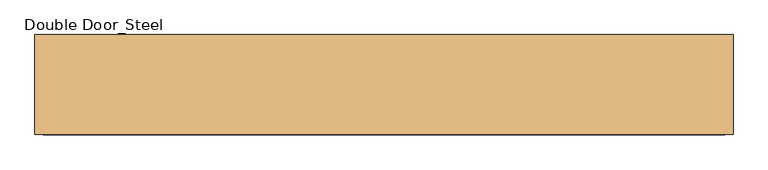
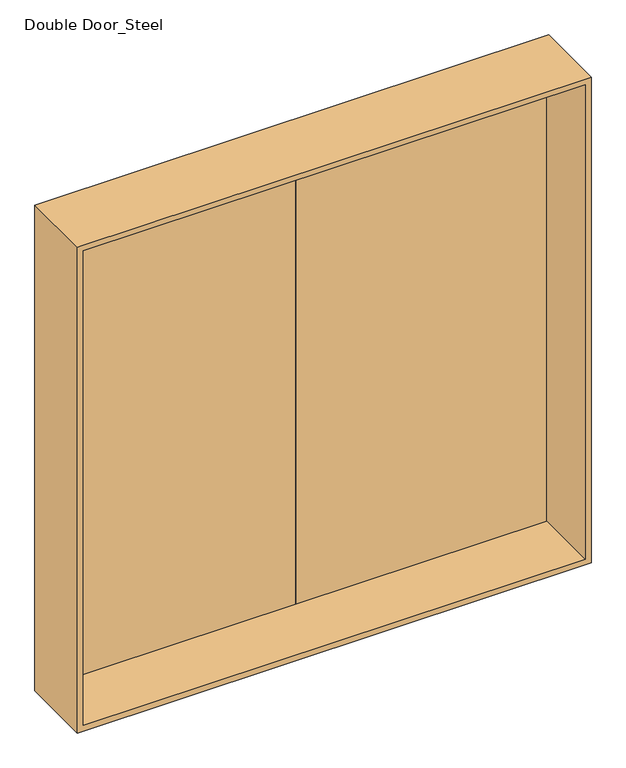
"""IFC4 building model written with IfcOpenShell, lengths in millimetres: door geometry, Double Door_Steel : H_DR_AMB_Double Door_Steel_W3000xH3000."""

from ifc_helpers import new_model, si_unit, frame, origin, place, context, project, spatial, polyline, outline, extrude, faceted_brep, source, transform, mapped, element, save


def double_door_steel_89dfd0fe(model_context):
    return source(origin(), model_context, "Body", "SolidModel", [
        extrude(outline(polyline([(1480.0, 175.0), (0.0, 175.0), (0.0, 215.0), (1480.0, 215.0), (1480.0, 175.0)])), frame((0.0, 0.0, 20.0), z_axis=(0.0, 0.0, 1.0), x_axis=(1.0, 0.0, 0.0)), (0.0, 0.0, 1.0), 2960.0),
        extrude(outline(polyline([(0.0, 175.0), (-1480.0, 175.0), (-1480.0, 215.0), (0.0, 215.0), (0.0, 175.0)])), frame((0.0, 0.0, 20.0), z_axis=(0.0, 0.0, 1.0), x_axis=(1.0, 0.0, 0.0)), (0.0, 0.0, 1.0), 2960.0),
        faceted_brep([(1500.0, -215.0, 3000.0), (1500.0, 215.0, 3000.0), (-1500.0, 215.0, 3000.0), (-1500.0, -215.0, 3000.0), (1465.0, 175.0, 2965.0), (1465.0, -215.0, 2965.0), (-1465.0, -215.0, 2965.0), (-1465.0, 175.0, 2965.0), (1480.0, 215.0, 2980.0), (1480.0, 175.0, 2980.0), (-1480.0, 175.0, 2980.0), (-1480.0, 215.0, 2980.0), (-1500.0, 215.0, 0.0), (-1500.0, -215.0, 0.0), (-1465.0, -215.0, 35.0), (-1465.0, 175.0, 35.0), (-1480.0, 175.0, 20.0), (-1480.0, 215.0, 20.0), (1500.0, 215.0, 0.0), (1480.0, 215.0, 20.0), (1500.0, -215.0, 0.0), (1465.0, -215.0, 35.0), (1465.0, 175.0, 35.0), (1480.0, 175.0, 20.0)], [[[0, 1, 2, 3]], [[4, 5, 6, 7]], [[8, 9, 10, 11]], [[3, 2, 12, 13]], [[7, 6, 14, 15]], [[11, 10, 16, 17]], [[18, 12, 2, 1], [8, 11, 17, 19]], [[13, 12, 18, 20]], [[0, 3, 13, 20], [21, 14, 6, 5]], [[15, 14, 21, 22]], [[23, 16, 10, 9], [4, 7, 15, 22]], [[17, 16, 23, 19]], [[20, 18, 1, 0]], [[22, 21, 5, 4]], [[19, 23, 9, 8]]]),
    ])


if __name__ == "__main__":
    model = new_model("IFC4")
    model_context = context("Model", 3, world=origin())
    ifc_project = project(units=[si_unit("LENGTHUNIT", "METRE", prefix="MILLI")], contexts=[model_context])
    site = spatial("IfcSite", under=ifc_project)
    building = spatial("IfcBuilding", under=site)
    placement = place(None, origin())
    double_door_steel_shape = double_door_steel_89dfd0fe(model_context)
    element("IfcDoor", 1, ObjectType="Double Door_Steel : H_DR_AMB_Double Door_Steel_W3000xH3000", at=placement, inside=building, context=model_context, shape_type="MappedRepresentation", body=[
        mapped(double_door_steel_shape, transform((0.0, 0.0, 0.0), x_axis=(1.0, 0.0, 0.0), y_axis=(0.0, 1.0, 0.0), z_axis=(0.0, 0.0, 1.0))),
    ])
    save(model, "model.ifc")

# Revit data of these elements
# Type "Double Door_Steel : H_DR_AMB_Double Door_Steel_W3000xH3000"
#   Type Mark = "362"
#   프레임 = ""
#   철물 = ""
#   유리/마감 = ""
#   위치/개소 = ""
#   부호 = "1/SD"
#   문번호 = ""
#   문기호 = "SD"
#   Analytic Construction = "<None>"
#   Height = 3000.000 mm
#   Width = 3000.000 mm
#   Define Thermal Properties by = 1
#   문 틀 = none
#   문 = none
#   Function = (empty or 0)
#   Assembly Code = ""
#   Wall Closure = (empty or 0)
